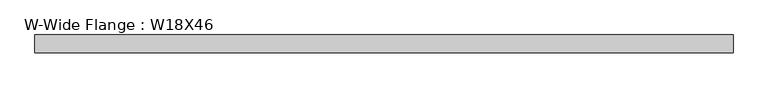
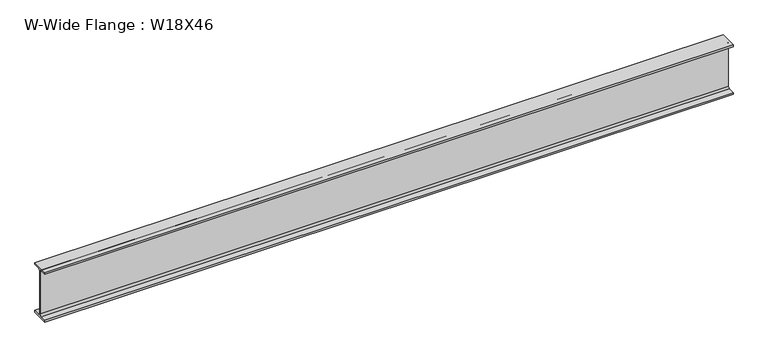
"""IFC4 building model written with IfcOpenShell, lengths in millimetres: beam geometry, W-Wide Flange : W18X46."""

from ifc_helpers import new_model, si_unit, point, frame, frame_2d, origin, place, context, project, spatial, polyline, circle_curve, trimmed, segment, composite_curve, outline, extrude, source, transform, mapped, element, save


def w_wide_flange_w18x46_bacc51cf(model_context):
    return source(origin(), model_context, "Body", "SweptSolid", [
        extrude(outline(composite_curve([segment(polyline([(76.962, -214.503), (76.962, -229.87), (-76.962, -229.87), (-76.962, -214.503), (-20.955, -214.503)]), True, "CONTINUOUS"), segment(trimmed(circle_curve(frame_2d((-20.955, -198.12)), 16.383), [point((-20.955, -214.503))], [point((-4.572, -198.12))], True, "CARTESIAN"), True, "CONTINUOUS"), segment(polyline([(-4.572, -198.12), (-4.572, 198.12)]), True, "CONTINUOUS"), segment(trimmed(circle_curve(frame_2d((-20.955, 198.12)), 16.383), [point((-4.572, 198.12))], [point((-20.955, 214.503))], True, "CARTESIAN"), True, "CONTINUOUS"), segment(polyline([(-20.955, 214.503), (-76.962, 214.503), (-76.962, 229.87), (76.962, 229.87), (76.962, 214.503), (20.955, 214.503)]), True, "CONTINUOUS"), segment(trimmed(circle_curve(frame_2d((20.955, 198.12)), 16.383), [point((20.955, 214.503))], [point((4.572, 198.12))], True, "CARTESIAN"), True, "CONTINUOUS"), segment(polyline([(4.572, 198.12), (4.572, -198.12)]), True, "CONTINUOUS"), segment(trimmed(circle_curve(frame_2d((20.955, -198.12)), 16.383), [point((4.572, -198.12))], [point((20.955, -214.503))], True, "CARTESIAN"), True, "CONTINUOUS"), segment(polyline([(20.955, -214.503), (76.962, -214.503)]), True, "CONTINUOUS")], self_intersect=False)), frame((-3035.3, 0.0, 0.0), z_axis=(1.0, 0.0, 0.0), x_axis=(0.0, 1.0, 0.0)), (0.0, 0.0, 1.0), 6070.6),
    ])


if __name__ == "__main__":
    model = new_model("IFC4")
    model_context = context("Model", 3, world=origin())
    ifc_project = project(units=[si_unit("LENGTHUNIT", "METRE", prefix="MILLI")], contexts=[model_context])
    site = spatial("IfcSite", under=ifc_project)
    building = spatial("IfcBuilding", under=site)
    placement = place(None, origin())
    w_wide_flange_w18x46_shape = w_wide_flange_w18x46_bacc51cf(model_context)
    element("IfcBeam", 1, ObjectType="W-Wide Flange : W18X46", at=placement, inside=building, context=model_context, shape_type="MappedRepresentation", body=[
        mapped(w_wide_flange_w18x46_shape, transform((0.0, 0.0, 0.0), x_axis=(1.0, 0.0, 0.0), y_axis=(0.0, 1.0, 0.0), z_axis=(0.0, 0.0, 1.0))),
    ])
    save(model, "model.ifc")

# Revit data of these elements
# Type "W-Wide Flange : W18X46"
#   Assembly Code = "B10"
#   W = 46
#   Length [instance default] = 5' - 0"
#   bf = 0' - 6.06"
#   d = 1' - 6.1"
#   k = 0' - 1 1/4"
#   k2 = 0' - 0.645"
#   tf = 0' - 0.605"
#   tw = 0' - 0.36"
#   A = 0.09375 SF
#   Structural Material [instance default] = Steel ASTM A992
# Element 1 (IfcBeam, "W-Wide Flange : W18X46")
#   Materials on its faces: "Steel ASTM A992"
# Materials
#   "Steel ASTM A992": class "Metal", colour RGB 199 199 199, transparency 0, Description = "Structural steel 50ksi", Cost = 0
